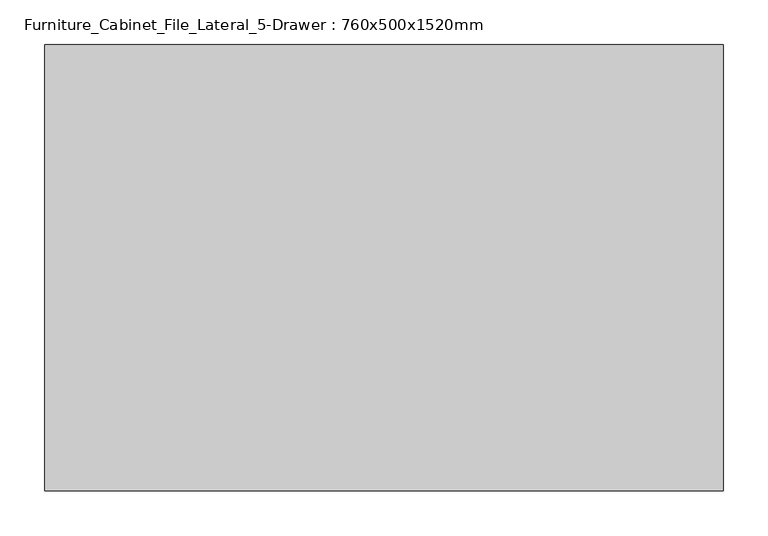
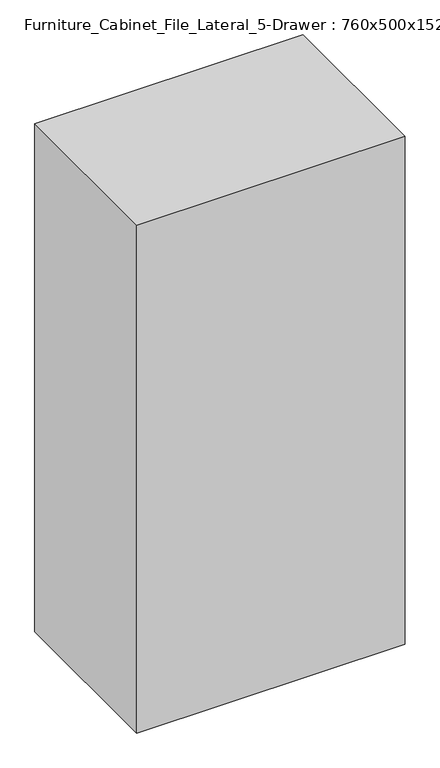
"""IFC4 building model written with IfcOpenShell, lengths in millimetres: furniture geometry, Furniture_Cabinet_File_Lateral_5-Drawer : 760x500x1520mm."""

from ifc_helpers import new_model, si_unit, frame, origin, place, context, project, spatial, polyline, outline, extrude, faceted_brep, source, transform, mapped, element, save


def furniture_cabinet_file_lateral_5_drawer_760x500x1520mm_cc6c2d8c(model_context):
    return source(origin(), model_context, "Body", "SolidModel", [
        extrude(outline(polyline([(76.2, -540.9725139), (76.2, 180.9274861), (361.15, 180.9274861), (361.15, -540.9725139), (76.2, -540.9725139)]), holes=[polyline([(335.75, -129.2225139), (297.65, -129.2225139), (297.65, -230.8225139), (335.75, -230.8225139), (335.75, -129.2225139)])]), frame((0.0, 1165.2683761, 0.0), z_axis=(0.0, 1.0, 0.0), x_axis=(0.0, 0.0, 1.0)), (0.0, 0.0, 1.0), 19.05),
        extrude(outline(polyline([(361.15, -540.9725139), (361.15, 180.9274861), (646.1, 180.9274861), (646.1, -540.9725139), (361.15, -540.9725139)]), holes=[polyline([(620.7, -129.2225139), (582.6, -129.2225139), (582.6, -230.8225139), (620.7, -230.8225139), (620.7, -129.2225139)])]), frame((0.0, 1165.2683761, 0.0), z_axis=(0.0, 1.0, 0.0), x_axis=(0.0, 0.0, 1.0)), (0.0, 0.0, 1.0), 19.05),
        extrude(outline(polyline([(1500.95, -540.9725139), (1216.0, -540.9725139), (1216.0, 180.9274861), (1500.95, 180.9274861), (1500.95, -540.9725139)]), holes=[polyline([(1241.4, -129.2225139), (1241.4, -230.8225139), (1279.5, -230.8225139), (1279.5, -129.2225139), (1241.4, -129.2225139)])]), frame((0.0, 1165.2683761, 0.0), z_axis=(0.0, 1.0, 0.0), x_axis=(0.0, 0.0, 1.0)), (0.0, 0.0, 1.0), 19.05),
        extrude(outline(polyline([(1216.0, -540.9725139), (931.05, -540.9725139), (931.05, 180.9274861), (1216.0, 180.9274861), (1216.0, -540.9725139)]), holes=[polyline([(1190.6, -129.2225139), (1152.5, -129.2225139), (1152.5, -230.8225139), (1190.6, -230.8225139), (1190.6, -129.2225139)])]), frame((0.0, 1165.2683761, 0.0), z_axis=(0.0, 1.0, 0.0), x_axis=(0.0, 0.0, 1.0)), (0.0, 0.0, 1.0), 19.05),
        extrude(outline(polyline([(931.05, -540.9725139), (646.1, -540.9725139), (646.1, 180.9274861), (931.05, 180.9274861), (931.05, -540.9725139)]), holes=[polyline([(905.65, -129.2225139), (867.55, -129.2225139), (867.55, -230.8225139), (905.65, -230.8225139), (905.65, -129.2225139)])]), frame((0.0, 1165.2683761, 0.0), z_axis=(0.0, 1.0, 0.0), x_axis=(0.0, 0.0, 1.0)), (0.0, 0.0, 1.0), 19.05),
        faceted_brep([(199.9774861, 684.3183761, 1520.0), (199.9774861, 1184.3183761, 1520.0), (-560.0225139, 1184.3183761, 1520.0), (-560.0225139, 684.3183761, 1520.0), (199.9774861, 684.3183761, 0.0), (-560.0225139, 684.3183761, 0.0), (-560.0225139, 1184.3183761, 0.0), (199.9774861, 1184.3183761, 0.0), (180.9274861, 1184.3183761, 76.2), (180.9274861, 1184.3183761, 1500.95), (-540.9725139, 1184.3183761, 1500.95), (-540.9725139, 1184.3183761, 76.2), (-540.9725139, 703.3683761, 76.2), (-540.9725139, 703.3683761, 1500.95), (180.9274861, 703.3683761, 1500.95), (180.9274861, 703.3683761, 76.2)], [[[0, 1, 2, 3]], [[4, 5, 6, 7]], [[3, 5, 4, 0]], [[2, 6, 5, 3]], [[1, 7, 6, 2], [8, 9, 10, 11]], [[0, 4, 7, 1]], [[12, 13, 14, 15]], [[15, 8, 11, 12]], [[14, 9, 8, 15]], [[13, 10, 9, 14]], [[12, 11, 10, 13]]]),
    ])


if __name__ == "__main__":
    model = new_model("IFC4")
    model_context = context("Model", 3, world=origin())
    ifc_project = project(units=[si_unit("LENGTHUNIT", "METRE", prefix="MILLI")], contexts=[model_context])
    site = spatial("IfcSite", under=ifc_project)
    building = spatial("IfcBuilding", under=site)
    placement = place(None, origin())
    furniture_cabinet_file_lateral_5_drawer_760x500x1520mm_shape = furniture_cabinet_file_lateral_5_drawer_760x500x1520mm_cc6c2d8c(model_context)
    element("IfcFurniture", 1, ObjectType="Furniture_Cabinet_File_Lateral_5-Drawer : 760x500x1520mm", at=placement, inside=building, context=model_context, shape_type="MappedRepresentation", body=[
        mapped(furniture_cabinet_file_lateral_5_drawer_760x500x1520mm_shape, transform((0.0, 0.0, 0.0), x_axis=(1.0, 0.0, 0.0), y_axis=(0.0, 1.0, 0.0), z_axis=(0.0, 0.0, 1.0))),
    ])
    save(model, "model.ifc")

# Revit data of these elements
# Type "Furniture_Cabinet_File_Lateral_5-Drawer : 760x500x1520mm"
#   Keynote = "N"
#   Assembly Code = "E2020200"
#   Depth = 500 mm
#   Height = 1520 mm
#   Width = 760 mm
#   Material = Metal - Steel
#   Default Elevation = 0
# Element 1 (IfcFurniture, "Furniture_Cabinet_File_Lateral_5-Drawer : 760x500x1520mm")
#   Materials on its faces: "Metal - Steel"
# Materials
#   "Metal - Steel": class "Metal", colour RGB 247 247 247, transparency 0
